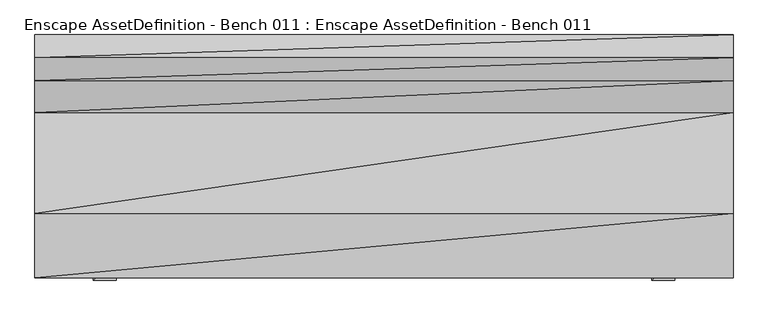
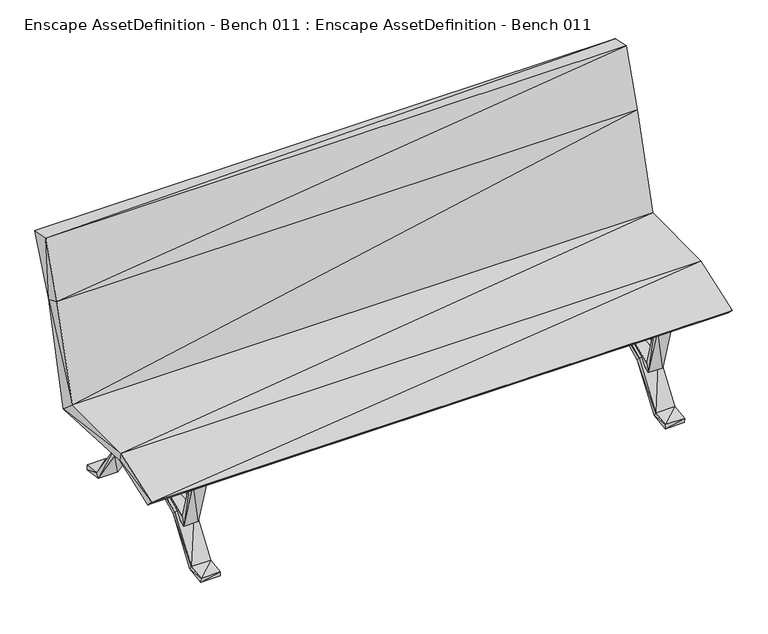
"""IFC4 building model written with IfcOpenShell, lengths in millimetres: geographic element geometry, Enscape AssetDefinition - Bench 011 : Enscape AssetDefinition - Bench 011."""

from ifc_helpers import new_model, si_unit, origin, place, context, project, spatial, faceted_brep, source, transform, mapped, element, save


def enscape_assetdefinition_bench_011_enscape_assetdefinition_35aa88c9(model_context):
    return source(origin(), model_context, "Body", "Brep", [
        faceted_brep([(861.7889881, -31.3537084, 209.5771432), (-853.7029624, -31.3537084, 209.5771432), (861.7889881, 40.1566327, 209.5771432), (-853.7029624, -31.3537084, 225.6669551), (861.7889881, -31.3537084, 225.6669551), (-853.7029624, 40.1566327, 209.5771432), (861.7889881, 40.1566327, 225.6669551), (-853.7029624, 40.1566327, 225.6669551)], [[[0, 1, 2]], [[3, 1, 4]], [[5, 1, 3]], [[2, 1, 5]], [[4, 1, 0]], [[6, 2, 7]], [[0, 2, 6]], [[7, 2, 5]], [[0, 6, 4]], [[6, 3, 4]], [[7, 3, 6]], [[5, 3, 7]]]),
        faceted_brep([(895.1288462, -192.6166713, 158.3775282), (823.6176372, 4.8564454, 251.7306805), (823.6176372, -192.6166713, 158.3775282), (895.1288462, 4.8564454, 251.7306805), (823.6176372, 202.3295611, 158.3775282), (823.6176372, 4.8564454, 233.8531017), (823.6176372, 190.7663345, 144.7431743), (823.6176372, -181.1052859, 144.6993798), (823.6176372, -298.276782, 8.243354), (895.1288462, -181.1052859, 144.6993798), (895.1288462, 4.8564454, 233.8531017), (823.6176372, -289.0206575, -7.0509193), (895.1288462, -298.276782, 8.2442481), (823.6176372, -360.8483374, 0.0), (895.1288462, -289.0206575, -7.0509193), (823.6176372, -358.5135043, -17.7247319), (895.1288462, -360.8483374, 0.0), (895.1288462, -358.5135043, -17.7247319), (895.1288462, 202.3295611, 158.3775282), (895.1288462, 307.0796728, 7.0974012), (895.1288462, 190.7663345, 144.7431743), (823.6176372, 297.9022264, -8.2451422), (823.6176372, 307.0796728, 7.0974012), (895.1288462, 369.6512282, 0.0), (895.1288462, 297.9022264, -8.2451422), (895.1288462, 367.6364422, -17.7640617), (823.6176372, 367.6364422, -17.7640617), (823.6176372, 369.6512282, 0.0)], [[[0, 1, 2]], [[3, 4, 1]], [[5, 2, 1]], [[6, 1, 4]], [[1, 0, 3]], [[1, 6, 5]], [[7, 8, 2]], [[8, 0, 2]], [[2, 5, 7]], [[5, 9, 7]], [[6, 10, 5]], [[9, 5, 10]], [[9, 11, 7]], [[8, 7, 11]], [[0, 8, 12]], [[11, 13, 8]], [[13, 12, 8]], [[11, 9, 14]], [[14, 15, 11]], [[13, 11, 15]], [[12, 13, 16]], [[15, 16, 13]], [[14, 0, 12]], [[17, 12, 16]], [[12, 17, 14]], [[15, 14, 17]], [[0, 14, 9]], [[16, 15, 17]], [[9, 3, 0]], [[10, 18, 3]], [[4, 3, 18]], [[3, 9, 10]], [[19, 4, 18]], [[20, 19, 18]], [[18, 10, 20]], [[21, 4, 22]], [[4, 19, 22]], [[4, 21, 6]], [[23, 22, 19]], [[24, 23, 19]], [[19, 20, 24]], [[6, 24, 20]], [[10, 6, 20]], [[24, 6, 21]], [[21, 25, 24]], [[25, 21, 26]], [[22, 26, 21]], [[26, 22, 27]], [[22, 23, 27]], [[25, 27, 23]], [[23, 24, 25]], [[27, 25, 26]]]),
        faceted_brep([(-821.1192489, -192.6166713, 158.3775282), (-892.6304579, 4.8564454, 251.7306805), (-892.6304579, -192.6166713, 158.3775282), (-821.1192489, 4.8564454, 251.7306805), (-892.6304579, 202.3295611, 158.3775282), (-892.6304579, 4.8564454, 233.8531017), (-892.6304579, 190.7663345, 144.7431743), (-892.6304579, -181.1052859, 144.6993798), (-892.6304579, -298.276782, 8.243354), (-821.1192489, -181.1052859, 144.6993798), (-821.1192489, 4.8564454, 233.8531017), (-892.6304579, -289.0206575, -7.0509193), (-821.1192489, -298.276782, 8.2442481), (-892.6295638, -360.8483374, 0.0), (-821.1192489, -289.0206575, -7.0509193), (-892.6295638, -358.5135043, -17.7247319), (-821.1192489, -360.8483374, 0.0), (-821.1192489, -358.5135043, -17.7247319), (-821.1192489, 202.3295611, 158.3775282), (-821.1192489, 307.0796728, 7.0974012), (-821.1192489, 190.7663345, 144.7431743), (-892.6304579, 297.9022264, -8.2451422), (-892.6304579, 307.0796728, 7.0974012), (-821.1192489, 369.6512282, 0.0), (-821.1192489, 297.9022264, -8.2451422), (-821.1192489, 367.6364422, -17.7640617), (-892.6295638, 367.6364422, -17.7640617), (-892.6295638, 369.6512282, 0.0)], [[[0, 1, 2]], [[3, 4, 1]], [[5, 2, 1]], [[6, 1, 4]], [[1, 0, 3]], [[1, 6, 5]], [[7, 8, 2]], [[8, 0, 2]], [[2, 5, 7]], [[5, 9, 7]], [[6, 10, 5]], [[9, 5, 10]], [[9, 11, 7]], [[8, 7, 11]], [[0, 8, 12]], [[11, 13, 8]], [[13, 12, 8]], [[11, 9, 14]], [[14, 15, 11]], [[13, 11, 15]], [[12, 13, 16]], [[15, 16, 13]], [[14, 0, 12]], [[17, 12, 16]], [[12, 17, 14]], [[15, 14, 17]], [[0, 14, 9]], [[16, 15, 17]], [[9, 3, 0]], [[10, 18, 3]], [[4, 3, 18]], [[3, 9, 10]], [[19, 4, 18]], [[20, 19, 18]], [[18, 10, 20]], [[21, 4, 22]], [[4, 19, 22]], [[4, 21, 6]], [[23, 22, 19]], [[24, 23, 19]], [[19, 20, 24]], [[6, 24, 20]], [[10, 6, 20]], [[24, 6, 21]], [[21, 25, 24]], [[25, 21, 26]], [[22, 26, 21]], [[26, 22, 27]], [[22, 23, 27]], [[25, 27, 23]], [[23, 24, 25]], [[27, 25, 26]]]),
        faceted_brep([(833.3135843, -224.7426957, 155.8451653), (886.9463205, -224.7426957, 155.8451653), (833.3135843, 4.8743235, 252.8659105), (886.9463205, -233.7878644, 123.4018132), (886.9463205, 4.8743235, 252.8659105), (886.9463205, -272.2845376, 316.5289164), (886.9463205, -293.8869298, 326.5295923), (833.3135843, -233.7878644, 123.4018132), (833.3135843, -272.2845376, 316.5289164), (886.9463205, -136.8117929, 354.6206653), (886.9463205, -138.1186396, 372.4901974), (833.3135843, -293.8869298, 326.5295923), (886.9463205, 206.2313557, 374.7874498), (833.3135843, -138.1186396, 372.4901974), (833.3135843, -136.8117929, 354.6206653), (886.9463205, 179.3711782, 356.7302227), (833.3135843, 134.3509406, 201.761052), (833.3135843, 206.2313557, 374.7874498), (886.9463205, 134.3509406, 201.761052), (833.3135843, 179.3711782, 356.7302227), (886.9463205, 124.2036298, 223.9355147), (833.3135843, 124.2036298, 223.9355147), (886.9463205, 4.8403558, 234.889105), (833.3135843, 4.8403558, 234.889105)], [[[0, 1, 2]], [[1, 3, 4]], [[0, 5, 1]], [[1, 6, 3]], [[2, 1, 4]], [[6, 1, 5]], [[7, 0, 2]], [[7, 8, 0]], [[5, 0, 8]], [[9, 10, 5]], [[8, 9, 5]], [[5, 10, 6]], [[11, 3, 6]], [[10, 11, 6]], [[9, 12, 10]], [[10, 13, 11]], [[12, 13, 10]], [[14, 15, 9]], [[14, 9, 8]], [[12, 9, 15]], [[12, 16, 17]], [[15, 18, 12]], [[12, 17, 13]], [[16, 12, 18]], [[19, 20, 15]], [[18, 15, 20]], [[15, 14, 19]], [[13, 19, 14]], [[13, 14, 8]], [[17, 21, 19]], [[20, 19, 21]], [[19, 13, 17]], [[13, 8, 11]], [[8, 7, 11]], [[3, 11, 7]], [[22, 3, 7]], [[7, 2, 23]], [[22, 7, 23]], [[4, 3, 22]], [[4, 22, 20]], [[22, 23, 16]], [[20, 22, 18]], [[22, 16, 18]], [[23, 2, 21]], [[23, 21, 16]], [[2, 4, 21]], [[21, 4, 20]], [[21, 17, 16]]]),
        faceted_brep([(-883.6907744, -224.7426957, 155.8451653), (-830.0580382, -224.7426957, 155.8451653), (-883.6907744, 4.8743235, 252.8659105), (-830.0580382, -233.7878644, 123.4018132), (-830.0580382, 4.8743235, 252.8659105), (-830.0580382, -272.2845376, 316.5289164), (-830.0580382, -293.8869298, 326.5295923), (-883.6907744, -233.7878644, 123.4018132), (-883.6907744, -272.2845376, 316.5289164), (-830.0580382, -136.8117929, 354.6206653), (-830.0580382, -138.1186396, 372.4901974), (-883.6907744, -293.8869298, 326.5295923), (-830.0580382, 206.2313557, 374.7874498), (-883.6907744, -138.1186396, 372.4901974), (-883.6907744, -136.8117929, 354.6206653), (-830.0580382, 179.3711782, 356.7302227), (-883.6907744, 134.3509406, 201.761052), (-883.6907744, 206.2313557, 374.7874498), (-830.0580382, 134.3509406, 201.761052), (-883.6907744, 179.3711782, 356.7302227), (-830.0580382, 124.2036298, 223.9355147), (-883.6907744, 124.2036298, 223.9355147), (-830.0580382, 4.8403558, 234.889105), (-883.6907744, 4.8403558, 234.889105)], [[[0, 1, 2]], [[1, 3, 4]], [[0, 5, 1]], [[1, 6, 3]], [[2, 1, 4]], [[6, 1, 5]], [[7, 0, 2]], [[7, 8, 0]], [[5, 0, 8]], [[9, 10, 5]], [[8, 9, 5]], [[5, 10, 6]], [[11, 3, 6]], [[10, 11, 6]], [[9, 12, 10]], [[10, 13, 11]], [[12, 13, 10]], [[14, 15, 9]], [[14, 9, 8]], [[12, 9, 15]], [[12, 16, 17]], [[15, 18, 12]], [[12, 17, 13]], [[16, 12, 18]], [[19, 20, 15]], [[18, 15, 20]], [[15, 14, 19]], [[13, 19, 14]], [[13, 14, 8]], [[17, 21, 19]], [[20, 19, 21]], [[19, 13, 17]], [[13, 8, 11]], [[8, 7, 11]], [[3, 11, 7]], [[22, 3, 7]], [[7, 2, 23]], [[22, 7, 23]], [[4, 3, 22]], [[4, 22, 20]], [[22, 23, 16]], [[20, 22, 18]], [[22, 16, 18]], [[23, 2, 21]], [[23, 21, 16]], [[2, 4, 21]], [[21, 4, 20]], [[21, 17, 16]]]),
        faceted_brep([(-1071.4054108, 393.8592672, 965.2250409), (-1071.4054108, 323.1480718, 979.290247), (1073.9047527, 393.8592672, 965.2250409), (-1071.4054108, 303.9877713, 750.4402399), (-1071.4054108, 252.6156306, 773.3073831), (1073.9047527, 323.1480718, 979.290247), (1073.9047527, 303.9877713, 750.4402399), (1073.9047527, 212.4303877, 377.7756989), (-1071.4054108, 212.4303877, 377.7756989), (-1071.4054108, 154.3246806, 429.0620089), (1073.9047527, 252.6156306, 773.3073831), (1073.9047527, 154.3246806, 429.0620089), (1073.9047527, -149.5084465, 394.7504759), (-1071.4054108, -149.5084465, 394.7504759), (-1071.4054108, -155.3660333, 427.3842275), (1073.9047527, -155.3660333, 427.3842275), (1073.9047527, -327.9222548, 329.6626508), (-1071.4054108, -327.9222548, 329.6626508), (-1071.4054108, -354.2899191, 354.8137248), (1073.9047527, -354.2899191, 354.8137248)], [[[0, 1, 2]], [[3, 4, 1]], [[2, 1, 5]], [[4, 5, 1]], [[3, 1, 0]], [[6, 0, 2]], [[5, 6, 2]], [[6, 3, 0]], [[7, 8, 3]], [[8, 9, 3]], [[7, 3, 6]], [[3, 9, 4]], [[4, 10, 5]], [[9, 10, 4]], [[10, 6, 5]], [[11, 7, 6]], [[11, 6, 10]], [[7, 11, 12]], [[12, 8, 7]], [[13, 14, 8]], [[12, 13, 8]], [[8, 14, 9]], [[9, 11, 10]], [[14, 11, 9]], [[14, 15, 11]], [[12, 11, 15]], [[12, 15, 16]], [[16, 13, 12]], [[17, 18, 13]], [[16, 17, 13]], [[13, 18, 14]], [[18, 15, 14]], [[18, 19, 15]], [[16, 15, 19]], [[16, 19, 17]], [[17, 19, 18]]]),
    ])


if __name__ == "__main__":
    model = new_model("IFC4")
    model_context = context("Model", 3, world=origin())
    ifc_project = project(units=[si_unit("LENGTHUNIT", "METRE", prefix="MILLI")], contexts=[model_context])
    site = spatial("IfcSite", under=ifc_project)
    building = spatial("IfcBuilding", under=site)
    placement = place(None, origin())
    enscape_assetdefinition_bench_011_enscape_assetdefinition_shape = enscape_assetdefinition_bench_011_enscape_assetdefinition_35aa88c9(model_context)
    element("IfcGeographicElement", 1, ObjectType="Enscape AssetDefinition - Bench 011 : Enscape AssetDefinition - Bench 011", at=placement, inside=building, context=model_context, shape_type="MappedRepresentation", body=[
        mapped(enscape_assetdefinition_bench_011_enscape_assetdefinition_shape, transform((0.0, 0.0, 0.0), x_axis=(1.0, 0.0, 0.0), y_axis=(0.0, 1.0, 0.0), z_axis=(0.0, 0.0, 1.0))),
    ])
    save(model, "model.ifc")

# Revit data of these elements
# Type "Enscape AssetDefinition - Bench 011 : Enscape AssetDefinition - Bench 011"
#   EnscapeAssetSource = "REMOTE"
#   EnscapeAssetId = "4bc0d6d9-ec32-4fa5-8aae-ebe81e52bea5"
#   Height = 0.97929 m
#   EnscapeNativeAssetHeight = 0.97929 m
#   Default Elevation = 0
